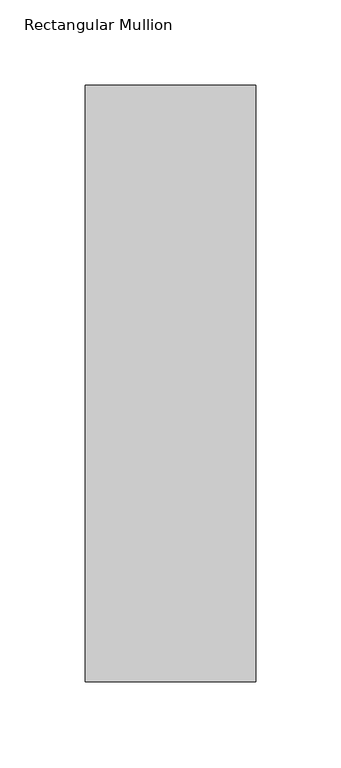
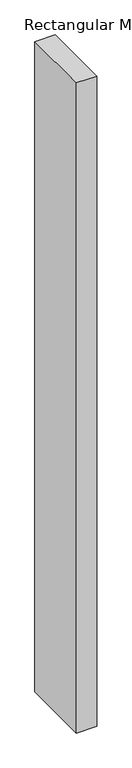
"""IFC4 building model written with IfcOpenShell, lengths in millimetres: member geometry, Rectangular Mullion : WWm-100x350-100mmOffset."""

from ifc_helpers import new_model, si_unit, frame, origin, place, context, project, spatial, polyline, outline, extrude, source, transform, mapped, element, save


def rectangular_mullion_ec13047d(model_context):
    return source(origin(), model_context, "Body", "SweptSolid", [
        extrude(outline(polyline([(0.0, 175.0), (0.0, -175.0), (-100.0, -175.0), (-100.0, 175.0), (0.0, 175.0)])), frame((0.0, 0.0, -3350.0), z_axis=(0.0, 0.0, 1.0), x_axis=(1.0, 0.0, 0.0)), (0.0, 0.0, 1.0), 3350.0),
    ])


if __name__ == "__main__":
    model = new_model("IFC4")
    model_context = context("Model", 3, world=origin())
    ifc_project = project(units=[si_unit("LENGTHUNIT", "METRE", prefix="MILLI")], contexts=[model_context])
    site = spatial("IfcSite", under=ifc_project)
    building = spatial("IfcBuilding", under=site)
    placement = place(None, origin())
    rectangular_mullion_shape = rectangular_mullion_ec13047d(model_context)
    element("IfcMember", 1, ObjectType="Rectangular Mullion : WWm-100x350-100mmOffset", at=placement, inside=building, context=model_context, shape_type="MappedRepresentation", body=[
        mapped(rectangular_mullion_shape, transform((0.0, 0.0, 0.0), x_axis=(1.0, 0.0, 0.0), y_axis=(0.0, 1.0, 0.0), z_axis=(0.0, 0.0, 1.0))),
    ])
    save(model, "model.ifc")

# Revit data of these elements
# Type "Rectangular Mullion : WWm-100x350-100mmOffset"
#   built-in parameter 1007304 = 1.14829 (stored number, unit not read)
#   built-in parameter 1007301 = 0.164042 (stored number, unit not read)
#   built-in parameter 1007300 = 0.164042 (stored number, unit not read)
# Element 1 (IfcMember, "Rectangular Mullion : WWm-100x350-100mmOffset")
#   Materials on its faces: "WW-EC-RGB-Mullion"
# Materials
#   "WW-EC-RGB-Mullion": class "Generic", colour RGB 255 255 255, transparency 0, Comments = "If region requests black mullions, switch asset color to RGB 25-25-25", Description = "Generic Color", Cost = 0
